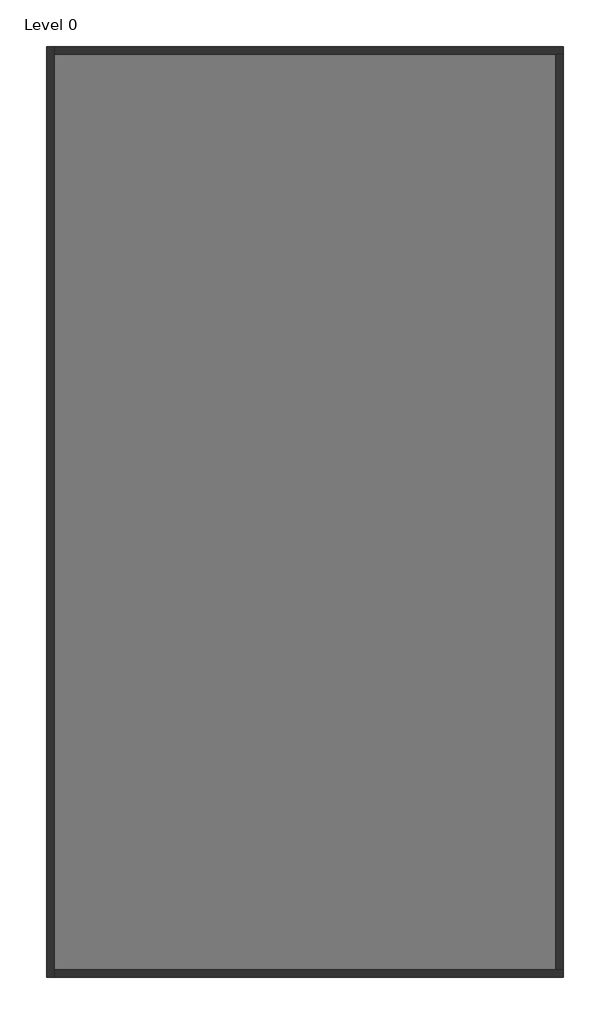
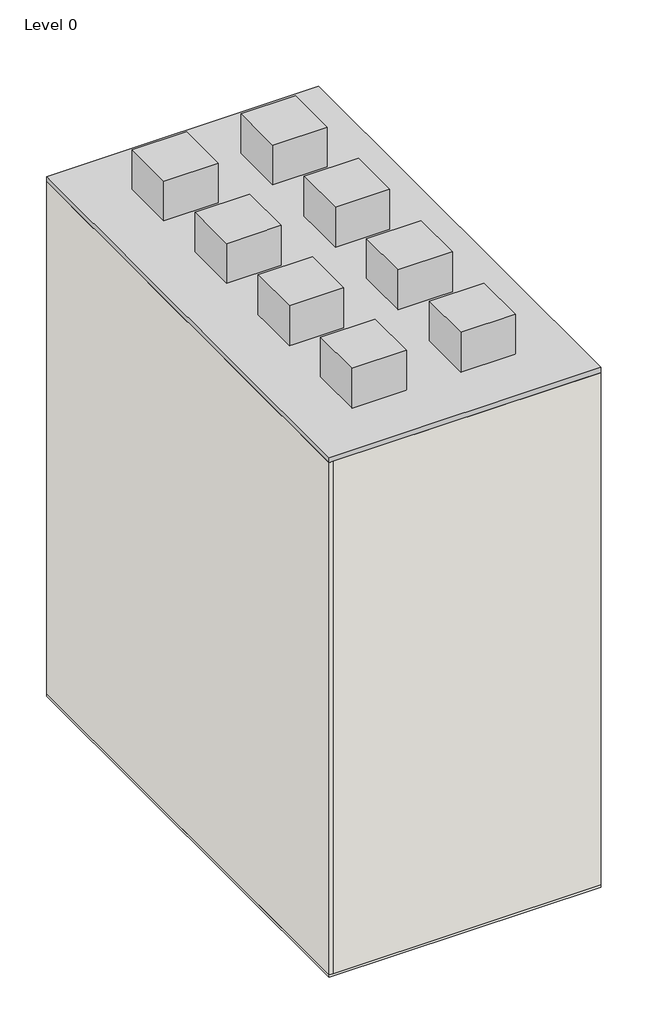
# One storey: 4 walls, 1 proxy, 1 slab.
"""IFC4 building model written with IfcOpenShell, lengths in millimetres."""

from ifc_helpers import new_model, si_unit, frame, origin, origin_with_axes, place, context, project, spatial, polyline, outline, extrude, faceted_brep, element, save

model = new_model("IFC4")

# Units and contexts
model_context = context("Model", 3, world=origin())
ifc_project = project(units=[si_unit("LENGTHUNIT", "METRE", prefix="MILLI")], contexts=[model_context])

# Site, building, storey
site = spatial("IfcSite", under=ifc_project)
building = spatial("IfcBuilding", under=site)
storey = spatial("IfcBuildingStorey", under=building, Name="Level 0", Elevation=100.0)

# Proxy
placement = place(None, origin())
element("IfcBuildingElementProxy", 1, Name="LowUrbanDensityBuilding : LowUrbanDensityBuilding", ObjectType="LowUrbanDensityBuilding : LowUrbanDensityBuilding", at=placement, inside=storey, context=model_context, shape_type="SweptSolid", body=[
    extrude(outline(polyline([(7325.2659446, 3676.2074539), (7325.2659446, -14323.7925461), (-2674.7340554, -14323.7925461), (-2674.7340554, 3676.2074539), (7325.2659446, 3676.2074539)])), origin_with_axes(), (0.0, 0.0, 1.0), 20200.0),
    extrude(outline(polyline([(1325.2659446, 1676.2074539), (1325.2659446, -323.7925461), (-674.7340554, -323.7925461), (-674.7340554, 1676.2074539), (1325.2659446, 1676.2074539)])), frame((0.0, 0.0, 20200.0), z_axis=(0.0, 0.0, 1.0), x_axis=(1.0, 0.0, 0.0)), (0.0, 0.0, 1.0), 1549.8),
    extrude(outline(polyline([(5325.2659446, 1676.2074539), (5325.2659446, -323.7925461), (3325.2659446, -323.7925461), (3325.2659446, 1676.2074539), (5325.2659446, 1676.2074539)])), frame((0.0, 0.0, 20200.0), z_axis=(0.0, 0.0, 1.0), x_axis=(1.0, 0.0, 0.0)), (0.0, 0.0, 1.0), 1549.8),
    extrude(outline(polyline([(1325.2659446, -2323.7925461), (1325.2659446, -4323.7925461), (-674.7340554, -4323.7925461), (-674.7340554, -2323.7925461), (1325.2659446, -2323.7925461)])), frame((0.0, 0.0, 20200.0), z_axis=(0.0, 0.0, 1.0), x_axis=(1.0, 0.0, 0.0)), (0.0, 0.0, 1.0), 1549.8),
    extrude(outline(polyline([(5325.2659446, -2323.7925461), (5325.2659446, -4323.7925461), (3325.2659446, -4323.7925461), (3325.2659446, -2323.7925461), (5325.2659446, -2323.7925461)])), frame((0.0, 0.0, 20200.0), z_axis=(0.0, 0.0, 1.0), x_axis=(1.0, 0.0, 0.0)), (0.0, 0.0, 1.0), 1549.8),
    extrude(outline(polyline([(1325.2659446, -6323.7925461), (1325.2659446, -8323.7925461), (-674.7340554, -8323.7925461), (-674.7340554, -6323.7925461), (1325.2659446, -6323.7925461)])), frame((0.0, 0.0, 20200.0), z_axis=(0.0, 0.0, 1.0), x_axis=(1.0, 0.0, 0.0)), (0.0, 0.0, 1.0), 1549.8),
    extrude(outline(polyline([(5325.2659446, -6323.7925461), (5325.2659446, -8323.7925461), (3325.2659446, -8323.7925461), (3325.2659446, -6323.7925461), (5325.2659446, -6323.7925461)])), frame((0.0, 0.0, 20200.0), z_axis=(0.0, 0.0, 1.0), x_axis=(1.0, 0.0, 0.0)), (0.0, 0.0, 1.0), 1549.8),
    extrude(outline(polyline([(1325.2659446, -10323.7925461), (1325.2659446, -12323.7925461), (-674.7340554, -12323.7925461), (-674.7340554, -10323.7925461), (1325.2659446, -10323.7925461)])), frame((0.0, 0.0, 20200.0), z_axis=(0.0, 0.0, 1.0), x_axis=(1.0, 0.0, 0.0)), (0.0, 0.0, 1.0), 1549.8),
    extrude(outline(polyline([(5325.2659446, -10323.7925461), (5325.2659446, -12323.7925461), (3325.2659446, -12323.7925461), (3325.2659446, -10323.7925461), (5325.2659446, -10323.7925461)])), frame((0.0, 0.0, 20200.0), z_axis=(0.0, 0.0, 1.0), x_axis=(1.0, 0.0, 0.0)), (0.0, 0.0, 1.0), 1549.8),
])

# Slab
element("IfcSlab", 2, ObjectType="Floor-Concrete_100Con", at=placement, inside=storey, context=model_context, shape_type="SweptSolid", body=[
    extrude(outline(polyline([(7325.2659446, 3676.2074539), (7325.2659446, -14323.7925461), (-2674.7340554, -14323.7925461), (-2674.7340554, 3676.2074539), (7325.2659446, 3676.2074539)])), origin_with_axes(), (0.0, 0.0, 1.0), 100.0),
])

# Walls
element("IfcWall", 3, ObjectType="Wall-Ext_25Rdr-100Blk-19P", at=placement, inside=storey, context=model_context, shape_type="Brep", body=[
    faceted_brep([(-2674.7340554, 3676.2074539, 100.0), (-2674.7340554, -14323.7925461, 100.0), (-2674.7340554, -14323.7925461, 20000.0), (-2674.7340554, 3676.2074539, 20000.0), (-2530.4340554, 3676.2074539, 100.0), (-2530.4340554, 3676.2074539, 20000.0), (-2530.4340554, 3531.9074539, 20000.0), (-2530.4340554, -14179.4925461, 20000.0), (-2530.4340554, -14323.7925461, 20000.0), (-2530.4340554, -14323.7925461, 100.0), (-2530.4340554, -14179.4925461, 100.0), (-2530.4340554, 3531.9074539, 100.0)], [[[0, 1, 2, 3]], [[4, 5, 6, 7, 8, 9, 10, 11]], [[1, 0, 4, 11, 10, 9]], [[3, 2, 8, 7, 6, 5]], [[2, 1, 9, 8]], [[0, 3, 5, 4]]]),
])
element("IfcWall", 4, ObjectType="Wall-Ext_25Rdr-100Blk-19P", at=placement, inside=storey, context=model_context, shape_type="Brep", body=[
    faceted_brep([(-2530.4340554, -14323.7925461, 100.0), (7325.2659446, -14323.7925461, 100.0), (7325.2659446, -14323.7925461, 20000.0), (-2530.4340554, -14323.7925461, 20000.0), (-2530.4340554, -14179.4925461, 100.0), (-2530.4340554, -14179.4925461, 20000.0), (7180.9659446, -14179.4925461, 20000.0), (7325.2659446, -14179.4925461, 20000.0), (7325.2659446, -14179.4925461, 100.0), (7180.9659446, -14179.4925461, 100.0)], [[[0, 1, 2, 3]], [[4, 5, 6, 7, 8, 9]], [[1, 0, 4, 9, 8]], [[3, 2, 7, 6, 5]], [[0, 3, 5, 4]], [[2, 1, 8, 7]]]),
])
element("IfcWall", 5, ObjectType="Wall-Ext_25Rdr-100Blk-19P", at=placement, inside=storey, context=model_context, shape_type="Brep", body=[
    faceted_brep([(7325.2659446, 3676.2074539, 100.0), (-2530.4340554, 3676.2074539, 100.0), (-2530.4340554, 3676.2074539, 20000.0), (7325.2659446, 3676.2074539, 20000.0), (7325.2659446, 3531.9074539, 100.0), (7325.2659446, 3531.9074539, 20000.0), (7180.9659446, 3531.9074539, 20000.0), (-2530.4340554, 3531.9074539, 20000.0), (-2530.4340554, 3531.9074539, 100.0), (7180.9659446, 3531.9074539, 100.0)], [[[0, 1, 2, 3]], [[4, 5, 6, 7, 8, 9]], [[1, 0, 4, 9, 8]], [[3, 2, 7, 6, 5]], [[2, 1, 8, 7]], [[0, 3, 5, 4]]]),
])
element("IfcWall", 6, ObjectType="Wall-Ext_25Rdr-100Blk-19P", at=placement, inside=storey, context=model_context, shape_type="SweptSolid", body=[
    extrude(outline(polyline([(7325.2659446, 3531.9074539), (7325.2659446, -14179.4925461), (7180.9659446, -14179.4925461), (7180.9659446, 3531.9074539), (7325.2659446, 3531.9074539)])), frame((0.0, 0.0, 100.0), z_axis=(0.0, 0.0, 1.0), x_axis=(1.0, 0.0, 0.0)), (0.0, 0.0, 1.0), 19900.0),
])

save(model, "model.ifc")

# Revit data of these elements
# Project information
#   Project Issue Date = "Issue Date"
#   Project Status = "Project Status"
#   Client Name = "Owner"
#   Project Address = "Enter address here"
#   Project Name = "Project Name"
#   Project Number = "Project Number"
# Type "Floor-Concrete_100Con"
#   Keynote = "E60/130"
#   Function = 0
#   Layers, outside or top first: 100 mm "Concrete" (function 1)
# Type "Wall-Ext_25Rdr-100Blk-19P"
#   Keynote = "F10"
#   Layers, outside or top first: 25.3 mm "Render, Beige, Smooth" (function 5); 100 mm "Concrete Masonry Units _Low Density" (function 1); 19 mm "Plaster" (function 5)
# Element 1 (IfcBuildingElementProxy, "LowUrbanDensityBuilding : LowUrbanDensityBuilding")
#   Phase Created = New Construction
#   Materials on its faces: "Default Form"
# Element 2 (IfcSlab, "Floor-Concrete_100Con")
#   Height Offset From Level = 0 mm
#   Phase Created = New Construction
#   Materials on its faces: "Concrete"
# Element 3 (IfcWall, "Wall-Ext_25Rdr-100Blk-19P")
#   Top Offset = 0 mm
#   Base Offset = 0 mm
#   wall height = 19900 mm
#   Phase Created = New Construction
#   Base Constraint = Level 0
#   Top Constraint = Level 5
#   Materials on its faces: "Render, Beige, Smooth", "Default Wall", "Plaster"
# Elements 4, 5, 6 (IfcWall, "Wall-Ext_25Rdr-100Blk-19P")
#   Top Offset = 0 mm
#   Base Offset = 0 mm
#   wall height = 19900 mm
#   Phase Created = New Construction
#   Base Constraint = Level 0
#   Top Constraint = Level 5
#   Materials on its faces: "Default Wall", "Render, Beige, Smooth", "Plaster"
# Materials
#   "Concrete": class "Concrete", colour RGB 120 120 120, transparency 0, Description = "Portland Cement Concrete", Cost = 0
#   "Render, Beige, Smooth": class "Generic", colour RGB 213 198 180, transparency 0, Description = "physical material", Cost = 0
#   "Concrete Masonry Units _Low Density": class "Masonry", colour RGB 181 181 181, transparency 0, Description = "Concrete masonry units", Cost = 0
#   "Plaster": class "Generic", colour RGB 249 249 249, transparency 0, Description = "Plaster", Cost = 0
#   "Default Form": class "Generic", colour RGB 185 189 196, transparency 0.5, Cost = 0
#   "Default Wall": class "Miscellaneous", colour RGB 128 128 128, transparency 0, Comments = "Rendering appearance not upgraded Rendering appearance not upgraded ", Cost = 0
